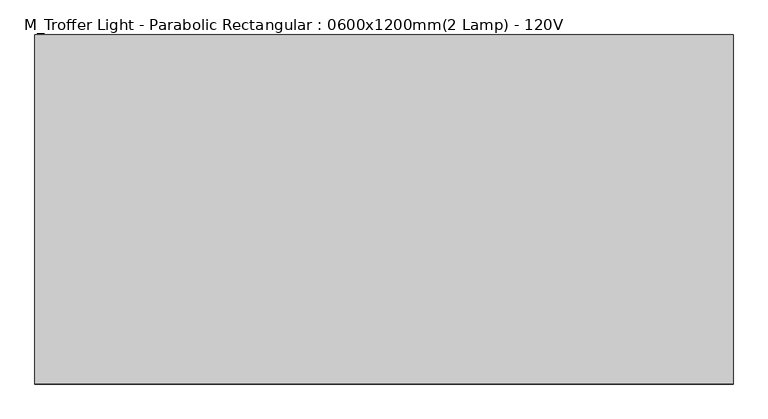
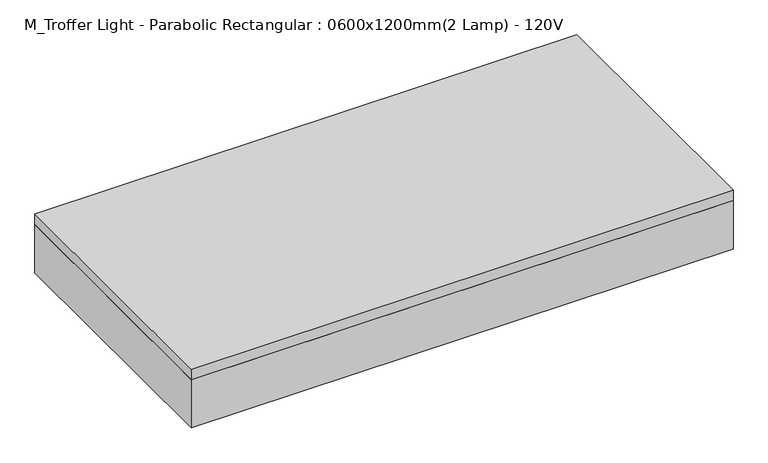
"""IFC4 building model written with IfcOpenShell, lengths in millimetres: light fixture geometry, M_Troffer Light - Parabolic Rectangular : 0600x1200mm(2 Lamp) - 120V."""

from ifc_helpers import new_model, si_unit, frame, origin, place, context, project, spatial, polyline, outline, extrude, source, transform, mapped, element, save


def m_troffer_light_parabolic_rectangular_0600x1200mm_2_lamp_ca384779(model_context):
    return source(origin(), model_context, "Body", "SweptSolid", [
        extrude(outline(polyline([(565.4964984, 219.9340679), (565.4964984, -338.8659321), (-602.9035016, -338.8659321), (-602.9035016, 219.9340679), (565.4964984, 219.9340679)]), holes=[polyline([(-409.2285016, 35.7840679), (-409.2285016, 213.5840679), (-596.5535016, 213.5840679), (-596.5535016, 35.7840679), (-409.2285016, 35.7840679)]), polyline([(-409.2285016, -148.3659321), (-409.2285016, 29.4340679), (-596.5535016, 29.4340679), (-596.5535016, -148.3659321), (-409.2285016, -148.3659321)]), polyline([(-409.2285016, -154.7159321), (-596.5535016, -154.7159321), (-596.5535016, -332.5159321), (-409.2285016, -332.5159321), (-409.2285016, -154.7159321)]), polyline([(-215.5535016, 35.7840679), (-215.5535016, 213.5840679), (-402.8785016, 213.5840679), (-402.8785016, 35.7840679), (-215.5535016, 35.7840679)]), polyline([(-215.5535016, -148.3659321), (-215.5535016, 29.4340679), (-402.8785016, 29.4340679), (-402.8785016, -148.3659321), (-215.5535016, -148.3659321)]), polyline([(-215.5535016, -154.7159321), (-402.8785016, -154.7159321), (-402.8785016, -332.5159321), (-215.5535016, -332.5159321), (-215.5535016, -154.7159321)]), polyline([(-21.8785016, 35.7840679), (-21.8785016, 213.5840679), (-209.2035016, 213.5840679), (-209.2035016, 35.7840679), (-21.8785016, 35.7840679)]), polyline([(-21.8785016, -148.3659321), (-21.8785016, 29.4340679), (-209.2035016, 29.4340679), (-209.2035016, -148.3659321), (-21.8785016, -148.3659321)]), polyline([(-21.8785016, -154.7159321), (-209.2035016, -154.7159321), (-209.2035016, -332.5159321), (-21.8785016, -332.5159321), (-21.8785016, -154.7159321)]), polyline([(171.7964984, 35.7840679), (171.7964984, 213.5840679), (-15.5285016, 213.5840679), (-15.5285016, 35.7840679), (171.7964984, 35.7840679)]), polyline([(171.7964984, -148.3659321), (171.7964984, 29.4340679), (-15.5285016, 29.4340679), (-15.5285016, -148.3659321), (171.7964984, -148.3659321)]), polyline([(171.7964984, -154.7159321), (-15.5285016, -154.7159321), (-15.5285016, -332.5159321), (171.7964984, -332.5159321), (171.7964984, -154.7159321)]), polyline([(365.4714984, 35.7840679), (365.4714984, 213.5840679), (178.1464984, 213.5840679), (178.1464984, 35.7840679), (365.4714984, 35.7840679)]), polyline([(365.4714984, -148.3659321), (365.4714984, 29.4340679), (178.1464984, 29.4340679), (178.1464984, -148.3659321), (365.4714984, -148.3659321)]), polyline([(365.4714984, -154.7159321), (178.1464984, -154.7159321), (178.1464984, -332.5159321), (365.4714984, -332.5159321), (365.4714984, -154.7159321)]), polyline([(559.1464984, 35.7840679), (559.1464984, 213.5840679), (371.8214984, 213.5840679), (371.8214984, 35.7840679), (559.1464984, 35.7840679)]), polyline([(559.1464984, -148.3659321), (559.1464984, 29.4340679), (371.8214984, 29.4340679), (371.8214984, -148.3659321), (559.1464984, -148.3659321)]), polyline([(559.1464984, -154.7159321), (371.8214984, -154.7159321), (371.8214984, -332.5159321), (559.1464984, -332.5159321), (559.1464984, -154.7159321)])]), frame((0.0, 0.0, 2438.4), z_axis=(0.0, 0.0, 1.0), x_axis=(1.0, 0.0, 0.0)), (0.0, 0.0, 1.0), 3.175),
        extrude(outline(polyline([(565.4964984, 219.9340679), (565.4964984, -338.8659321), (-602.9035016, -338.8659321), (-602.9035016, 219.9340679), (565.4964984, 219.9340679)])), frame((0.0, 0.0, 2514.6), z_axis=(0.0, 0.0, 1.0), x_axis=(1.0, 0.0, 0.0)), (0.0, 0.0, 1.0), 6.35),
        extrude(outline(polyline([(565.4964984, 219.9340679), (565.4964984, -338.8659321), (-602.9035016, -338.8659321), (-602.9035016, 219.9340679), (565.4964984, 219.9340679)]), holes=[polyline([(-409.2285016, 35.7840679), (-409.2285016, 213.5840679), (-596.5535016, 213.5840679), (-596.5535016, 35.7840679), (-409.2285016, 35.7840679)]), polyline([(-409.2285016, -148.3659321), (-409.2285016, 29.4340679), (-596.5535016, 29.4340679), (-596.5535016, -148.3659321), (-409.2285016, -148.3659321)]), polyline([(-409.2285016, -154.7159321), (-596.5535016, -154.7159321), (-596.5535016, -332.5159321), (-409.2285016, -332.5159321), (-409.2285016, -154.7159321)]), polyline([(-215.5535016, 35.7840679), (-215.5535016, 213.5840679), (-402.8785016, 213.5840679), (-402.8785016, 35.7840679), (-215.5535016, 35.7840679)]), polyline([(-215.5535016, -148.3659321), (-215.5535016, 29.4340679), (-402.8785016, 29.4340679), (-402.8785016, -148.3659321), (-215.5535016, -148.3659321)]), polyline([(-215.5535016, -154.7159321), (-402.8785016, -154.7159321), (-402.8785016, -332.5159321), (-215.5535016, -332.5159321), (-215.5535016, -154.7159321)]), polyline([(-21.8785016, 35.7840679), (-21.8785016, 213.5840679), (-209.2035016, 213.5840679), (-209.2035016, 35.7840679), (-21.8785016, 35.7840679)]), polyline([(-21.8785016, -148.3659321), (-21.8785016, 29.4340679), (-209.2035016, 29.4340679), (-209.2035016, -148.3659321), (-21.8785016, -148.3659321)]), polyline([(-21.8785016, -154.7159321), (-209.2035016, -154.7159321), (-209.2035016, -332.5159321), (-21.8785016, -332.5159321), (-21.8785016, -154.7159321)]), polyline([(171.7964984, 35.7840679), (171.7964984, 213.5840679), (-15.5285016, 213.5840679), (-15.5285016, 35.7840679), (171.7964984, 35.7840679)]), polyline([(171.7964984, -148.3659321), (171.7964984, 29.4340679), (-15.5285016, 29.4340679), (-15.5285016, -148.3659321), (171.7964984, -148.3659321)]), polyline([(171.7964984, -154.7159321), (-15.5285016, -154.7159321), (-15.5285016, -332.5159321), (171.7964984, -332.5159321), (171.7964984, -154.7159321)]), polyline([(365.4714984, 35.7840679), (365.4714984, 213.5840679), (178.1464984, 213.5840679), (178.1464984, 35.7840679), (365.4714984, 35.7840679)]), polyline([(365.4714984, -148.3659321), (365.4714984, 29.4340679), (178.1464984, 29.4340679), (178.1464984, -148.3659321), (365.4714984, -148.3659321)]), polyline([(365.4714984, -154.7159321), (178.1464984, -154.7159321), (178.1464984, -332.5159321), (365.4714984, -332.5159321), (365.4714984, -154.7159321)]), polyline([(559.1464984, 35.7840679), (559.1464984, 213.5840679), (371.8214984, 213.5840679), (371.8214984, 35.7840679), (559.1464984, 35.7840679)]), polyline([(559.1464984, -148.3659321), (559.1464984, 29.4340679), (371.8214984, 29.4340679), (371.8214984, -148.3659321), (559.1464984, -148.3659321)]), polyline([(559.1464984, -154.7159321), (371.8214984, -154.7159321), (371.8214984, -332.5159321), (559.1464984, -332.5159321), (559.1464984, -154.7159321)])]), frame((0.0, 0.0, 2441.575), z_axis=(0.0, 0.0, 1.0), x_axis=(1.0, 0.0, 0.0)), (0.0, 0.0, 1.0), 47.625),
        extrude(outline(polyline([(590.8964984, 245.3340679), (590.8964984, -364.2659321), (-628.3035016, -364.2659321), (-628.3035016, 245.3340679), (590.8964984, 245.3340679)]), holes=[polyline([(565.4964984, 219.9340679), (-602.9035016, 219.9340679), (-602.9035016, -338.8659321), (565.4964984, -338.8659321), (565.4964984, 219.9340679)])]), frame((0.0, 0.0, 2438.4), z_axis=(0.0, 0.0, 1.0), x_axis=(1.0, 0.0, 0.0)), (0.0, 0.0, 1.0), 114.3),
        extrude(outline(polyline([(590.8964984, 245.3340679), (590.8964984, -364.2659321), (-628.3035016, -364.2659321), (-628.3035016, 245.3340679), (590.8964984, 245.3340679)])), frame((0.0, 0.0, 2552.7), z_axis=(0.0, 0.0, 1.0), x_axis=(1.0, 0.0, 0.0)), (0.0, 0.0, 1.0), 25.4),
    ])


if __name__ == "__main__":
    model = new_model("IFC4")
    model_context = context("Model", 3, world=origin())
    ifc_project = project(units=[si_unit("LENGTHUNIT", "METRE", prefix="MILLI")], contexts=[model_context])
    site = spatial("IfcSite", under=ifc_project)
    building = spatial("IfcBuilding", under=site)
    placement = place(None, origin())
    m_troffer_light_parabolic_rectangular_0600x1200mm_2_lamp_shape = m_troffer_light_parabolic_rectangular_0600x1200mm_2_lamp_ca384779(model_context)
    element("IfcLightFixture", 1, ObjectType="M_Troffer Light - Parabolic Rectangular : 0600x1200mm(2 Lamp) - 120V", at=placement, inside=building, context=model_context, shape_type="MappedRepresentation", body=[
        mapped(m_troffer_light_parabolic_rectangular_0600x1200mm_2_lamp_shape, transform((0.0, 0.0, 0.0), x_axis=(1.0, 0.0, 0.0), y_axis=(0.0, 1.0, 0.0), z_axis=(0.0, 0.0, 1.0))),
    ])
    save(model, "model.ifc")

# Revit data of these elements
# Type "M_Troffer Light - Parabolic Rectangular : 0600x1200mm(2 Lamp) - 120V"
#   Assembly Code = "D5020210"
#   Lamp = "T-12"
#   Wattage = 80 W
#   built-in parameter 1150110 = 1 (stored number, unit not read)
#   built-in parameter 1114217 = 0.88 (stored number, unit not read)
#   built-in parameter 1150109 = 1 (stored number, unit not read)
#   built-in parameter 1150113 = 1 (stored number, unit not read)
#   built-in parameter 1150115 = 1 (stored number, unit not read)
#   built-in parameter 1150105 = 2005.35 (stored number, unit not read)
#   Light Source Symbol Size = 609.6 mm
#   built-in parameter 1150112 = 1 (stored number, unit not read)
#   built-in parameter 1150114 = 1 (stored number, unit not read)
#   built-in parameter 1150107 = 4230 (stored number, unit not read)
#   built-in parameter 1150106 = 20.0535 (stored number, unit not read)
#   Emit from Rectangle Width = 550 mm
#   Emit from Rectangle Length = 1150 mm
#   built-in parameter 1150104 = 7.31611 (stored number, unit not read)
#   Ballast Voltage = 120 V
#   built-in parameter 1114218 = 0.88 (stored number, unit not read)
#   built-in parameter 1150133 = 10 (stored number, unit not read)
#   Lumens = 6300 lm
#   Apparent Load = 80 VA
#   built-in parameter 1150134 = 8
#   built-in parameter 1150137 = 1
#   Color Filter = 16777215
#   built-in parameter 1140040 [instance default] = 1
#   Ballast Number of Poles = 1
#   Load Classification = Lighting - Dwelling Unit
#   Grid Material = Metal - Paint Finish - Dark Gray, Matte
#   Diffuser Material = Glass - White, High Luminance
#   Light Box Material = Metal - Chrome
#   Emit Shape Visible in Rendering = no
#   Dimming Lamp Color Temperature Shift = (empty or 0)
#   Default Elevation = 0
#   Wattage Comments = ""
# Element 1 (IfcLightFixture, "M_Troffer Light - Parabolic Rectangular : 0600x1200mm(2 Lamp) - 120V")
#   Materials on its faces: "Glass - White, High Luminance", "Metal - Paint Finish - Dark Gray, Matte", "Metal - Chrome"
# Materials
#   "Metal - Paint Finish - Dark Gray, Matte": class "Paint", colour RGB 98 98 98, transparency 0
#   "Glass - White, High Luminance": class "Glass", colour RGB 249 250 249, transparency 0.8
#   "Metal - Chrome": class "Metal", colour RGB 17 17 17, transparency 0
